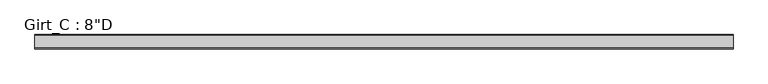
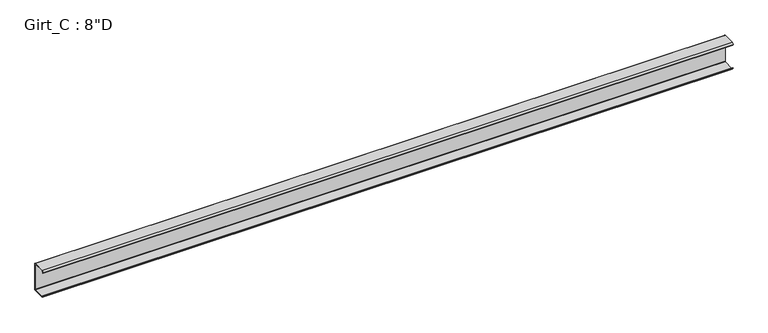
"""IFC4 building model written with IfcOpenShell, lengths in millimetres: beam geometry."""

from ifc_helpers import new_model, si_unit, point, frame, frame_2d, origin, place, context, project, spatial, polyline, circle_curve, trimmed, segment, composite_curve, outline, extrude, source, transform, mapped, element, save


def beam_31f30789(model_context):
    return source(origin(), model_context, "Body", "SweptSolid", [
        extrude(outline(composite_curve([segment(polyline([(-87.5109375, 101.6), (-3.3734375, 101.6)]), True, "CONTINUOUS"), segment(trimmed(circle_curve(frame_2d((-3.3734375, 96.8375)), 4.7625), [point((-3.3734375, 101.6))], [point((1.3890625, 96.8375))], False, "CARTESIAN"), True, "CONTINUOUS"), segment(polyline([(1.3890625, 96.8375), (1.3890625, -96.8375)]), True, "CONTINUOUS"), segment(trimmed(circle_curve(frame_2d((-3.3734375, -96.8375)), 4.7625), [point((1.3890625, -96.8375))], [point((-3.3734375, -101.6))], False, "CARTESIAN"), True, "CONTINUOUS"), segment(polyline([(-3.3734375, -101.6), (-87.5109375, -101.6), (-99.7792647, -86.979177), (-97.6510975, -85.1934327), (-86.2154765, -98.821875), (-3.2694106, -98.821875)]), True, "CONTINUOUS"), segment(trimmed(circle_curve(frame_2d((-3.3748024, -96.8389339)), 1.9857399), [point((-3.2694106, -98.821875))], [point((-1.3890625, -96.8389339))], True, "CARTESIAN"), True, "CONTINUOUS"), segment(polyline([(-1.3890625, -96.8389339), (-1.3890625, 96.8381931)]), True, "CONTINUOUS"), segment(trimmed(circle_curve(frame_2d((-3.3741066, 96.8381931)), 1.9850441), [point((-1.3890625, 96.8381931))], [point((-3.3005807, 98.821875))], True, "CARTESIAN"), True, "CONTINUOUS"), segment(polyline([(-3.3005807, 98.821875), (-86.2154765, 98.821875), (-97.6278742, 85.221109), (-99.7560415, 87.0068534), (-87.5109375, 101.6)]), True, "CONTINUOUS")], self_intersect=False)), frame((-2429.66875, 0.0, 0.0), z_axis=(1.0, 0.0, 0.0), x_axis=(0.0, 1.0, 0.0)), (0.0, 0.0, 1.0), 4914.2015),
    ])


if __name__ == "__main__":
    model = new_model("IFC4")
    model_context = context("Model", 3, world=origin())
    ifc_project = project(units=[si_unit("LENGTHUNIT", "METRE", prefix="MILLI")], contexts=[model_context])
    site = spatial("IfcSite", under=ifc_project)
    building = spatial("IfcBuilding", under=site)
    placement = place(None, origin())
    beam_shape = beam_31f30789(model_context)
    element("IfcBeam", 1, ObjectType="Girt_C : 8\"D", at=placement, inside=building, context=model_context, shape_type="MappedRepresentation", body=[
        mapped(beam_shape, transform((0.0, 0.0, 0.0), x_axis=(1.0, 0.0, 0.0), y_axis=(0.0, 1.0, 0.0), z_axis=(0.0, 0.0, 1.0))),
    ])
    save(model, "model.ifc")

# Revit data of these elements
# Type "Girt_C : 8\"D"
#   half leg = 0' - 1 3/4"
#   Web_Thickness = 0' - 0 7/64"
#   Length [instance default] = 10' - 0"
#   Leg_1 = 0' - 3 1/2"
#   Height = 0' - 8"
#   Structural Material [instance default] = none
# Element 1 (IfcBeam, "Girt_C : 8\"D")
#   Structural Material = CEE' SECTION (8.0x3.5C - SEE STRUCT. DWGS)
#   Materials on its faces: "CEE' SECTION (8.0x3.5C - SEE STRUCT. DWGS)"
# Materials
#   "CEE' SECTION (8.0x3.5C - SEE STRUCT. DWGS)": class "Metal", colour RGB 137 146 153, transparency 0, Description = "Steel, mill finish", Cost = 0
